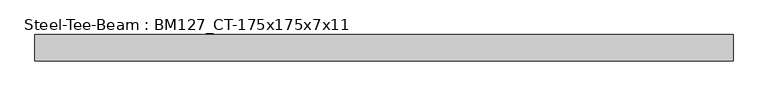
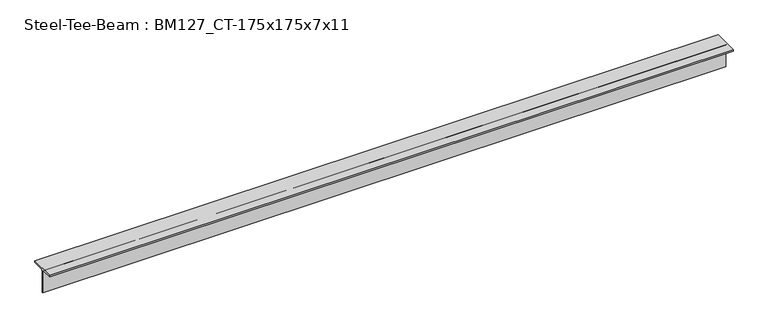
"""IFC4 building model written with IfcOpenShell, lengths in millimetres: beam geometry, Steel-Tee-Beam : BM127_CT-175x175x7x11."""

import ifcopenshell
import ifcopenshell.guid

model = None  # the IFC model being written
_history = None  # IfcOwnerHistory: only IFC2X3 demands one
_inside = {}  # id of a spatial element -> (the spatial element, [elements in it])
_under = {}  # id of a project, library or spatial element -> (it, [spatial elements below it])
_declared = {}  # id of a project -> (the project, [libraries it declares])
_typed = {}  # id of a type object -> (the type object, [elements of that type])
_made_of = {}  # id of a material, layer set ... -> (it, [elements and type objects made of it])


def new_model(schema):
    """Start an empty IFC model of exactly this schema.

    Asked for "IFC4X3", IfcOpenShell would pick the latest addendum, in which some entities
    have other attributes; the version numbers below select the first issue.
    IFC2X3 requires an IfcOwnerHistory on every rooted entity: one is made here for all.
    """
    global model, _history
    if schema == "IFC4X3":
        model = ifcopenshell.file(schema_version=(4, 3, 0, 0))
    else:
        model = ifcopenshell.file(schema=schema)
    _inside.clear()
    _under.clear()
    _declared.clear()
    _typed.clear()
    _made_of.clear()
    _history = None
    if model.schema == "IFC2X3":
        org = make("IfcOrganization", Name="unknown")
        user = make(
            "IfcPersonAndOrganization",
            ThePerson=make("IfcPerson", FamilyName="unknown"),
            TheOrganization=org,
        )
        app = make(
            "IfcApplication",
            ApplicationDeveloper=org,
            Version="unknown",
            ApplicationFullName="unknown",
            ApplicationIdentifier="unknown",
        )
        _history = make(
            "IfcOwnerHistory",
            OwningUser=user,
            OwningApplication=app,
            ChangeAction="ADDED",
            CreationDate=0,
        )
    return model


def make(cls, **values):
    """One entity of the class cls with the attributes given. An attribute that is None is left unset."""
    return model.create_entity(
        cls, **{name: value for name, value in values.items() if value is not None}
    )


def rooted(cls, **values):
    """An entity with a GlobalId (a new one), such as an element, a storey or a relation."""
    return make(cls, GlobalId=ifcopenshell.guid.new(), OwnerHistory=_history, **values)


def si_unit(unit_type, name, prefix=None):
    """IfcSIUnit, for example si_unit("LENGTHUNIT", "METRE", prefix="MILLI")."""
    return make("IfcSIUnit", UnitType=unit_type, Prefix=prefix, Name=name)


def assignment(units):
    """IfcUnitAssignment: the units of a project."""
    return None if units is None else make("IfcUnitAssignment", Units=units)


def point(xyz):
    """IfcCartesianPoint."""
    return None if xyz is None else make("IfcCartesianPoint", Coordinates=xyz)


def direction(xyz):
    """IfcDirection."""
    return None if xyz is None else make("IfcDirection", DirectionRatios=xyz)


def frame(location, z_axis=None, x_axis=None):
    """IfcAxis2Placement3D, a coordinate frame: its origin and axes. An axis left out is left unset."""
    return make(
        "IfcAxis2Placement3D",
        Location=point(location),
        Axis=direction(z_axis),
        RefDirection=direction(x_axis),
    )


def frame_2d(location, x_axis=None):
    """IfcAxis2Placement2D, a coordinate frame in the plane: its origin and x axis."""
    return make(
        "IfcAxis2Placement2D", Location=point(location), RefDirection=direction(x_axis)
    )


def origin():
    """The frame at (0, 0, 0) with its axes left unset."""
    return frame((0.0, 0.0, 0.0))


def place(relative_to, where):
    """IfcLocalPlacement: puts the frame where relative to a parent placement (None: the world)."""
    return make(
        "IfcLocalPlacement", PlacementRelTo=relative_to, RelativePlacement=where
    )


def context(
    kind, dimensions, precision=None, world=None, true_north=None, identifier=None
):
    """IfcGeometricRepresentationContext, for example the 3D "Model" context."""
    return make(
        "IfcGeometricRepresentationContext",
        ContextIdentifier=identifier,
        ContextType=kind,
        CoordinateSpaceDimension=dimensions,
        Precision=precision,
        WorldCoordinateSystem=world,
        TrueNorth=true_north,
    )


def project(units=None, contexts=None):
    """IfcProject with its units and contexts."""
    return rooted(
        "IfcProject",
        Name="project",
        RepresentationContexts=contexts,
        UnitsInContext=assignment(units),
    )


def spatial(cls, under=None, at=None, **own):
    """A site, building, storey or space (cls), placed at a placement, below another one or the project."""
    s = rooted(cls, ObjectPlacement=at, **own)
    if under is not None:
        _under.setdefault(under.id(), (under, []))[1].append(s)
    return s


def polyline(points):
    """IfcPolyline through the points."""
    return make("IfcPolyline", Points=[point(p) for p in points])


def circle_curve(where, radius):
    """IfcCircle in the frame where."""
    return make("IfcCircle", Position=where, Radius=radius)


def trimmed(basis, trim1, trim2, sense, master):
    """IfcTrimmedCurve: the piece of a basis curve between two trims."""
    return make(
        "IfcTrimmedCurve",
        BasisCurve=basis,
        Trim1=trim1,
        Trim2=trim2,
        SenseAgreement=sense,
        MasterRepresentation=master,
    )


def segment(curve, same_sense, transition):
    """IfcCompositeCurveSegment."""
    return make(
        "IfcCompositeCurveSegment",
        Transition=transition,
        SameSense=same_sense,
        ParentCurve=curve,
    )


def composite_curve(segments, self_intersect=None):
    """IfcCompositeCurve: segments joined end to end."""
    return make("IfcCompositeCurve", Segments=segments, SelfIntersect=self_intersect)


def outline(outer, holes=None, kind="AREA"):
    """IfcArbitraryClosedProfileDef: a profile drawn as a closed curve; with holes, ...WithVoids."""
    if holes is None:
        return make("IfcArbitraryClosedProfileDef", ProfileType=kind, OuterCurve=outer)
    return make(
        "IfcArbitraryProfileDefWithVoids",
        ProfileType=kind,
        OuterCurve=outer,
        InnerCurves=holes,
    )


def extrude(swept, where, along, depth):
    """IfcExtrudedAreaSolid: the profile swept, set in the frame where, extruded along a direction by depth."""
    return make(
        "IfcExtrudedAreaSolid",
        SweptArea=swept,
        Position=where,
        ExtrudedDirection=direction(along),
        Depth=depth,
    )


def shape(context_of_items, identifier, shape_type, items):
    """IfcShapeRepresentation: the items that make up one representation, for example the "Body"."""
    return make(
        "IfcShapeRepresentation",
        ContextOfItems=context_of_items,
        RepresentationIdentifier=identifier,
        RepresentationType=shape_type,
        Items=items,
    )


def source(mapping_origin, context_of_items, identifier, shape_type, items):
    """IfcRepresentationMap: a shape defined once, which mapped items show again and again."""
    return make(
        "IfcRepresentationMap",
        MappingOrigin=mapping_origin,
        MappedRepresentation=shape(context_of_items, identifier, shape_type, items),
    )


def transform(
    local_origin,
    x_axis=None,
    y_axis=None,
    z_axis=None,
    scale=None,
    scale2=None,
    scale3=None,
    uniform=True,
):
    """IfcCartesianTransformationOperator3D, or its non-uniform kind. x_axis, y_axis, z_axis: its Axis1, 2, 3."""
    if uniform:
        return make(
            "IfcCartesianTransformationOperator3D",
            Axis1=direction(x_axis),
            Axis2=direction(y_axis),
            LocalOrigin=point(local_origin),
            Scale=scale,
            Axis3=direction(z_axis),
        )
    return make(
        "IfcCartesianTransformationOperator3DnonUniform",
        Axis1=direction(x_axis),
        Axis2=direction(y_axis),
        LocalOrigin=point(local_origin),
        Scale=scale,
        Axis3=direction(z_axis),
        Scale2=scale2,
        Scale3=scale3,
    )


def mapped(mapping_source, mapping_target):
    """IfcMappedItem: shows the shape of a source again, moved by a transform."""
    return make(
        "IfcMappedItem", MappingSource=mapping_source, MappingTarget=mapping_target
    )


def made_of(thing, what):
    """Note that an element or type object is made of a material, layer set ...; save() writes the relation."""
    if what is not None:
        _made_of.setdefault(what.id(), (what, []))[1].append(thing)
    return thing


def element(
    cls,
    number,
    at=None,
    inside=None,
    cuts=None,
    type_object=None,
    material=None,
    context=None,
    identifier="Body",
    shape_type=None,
    held_by="IfcProductDefinitionShape",
    body=None,
    shapes=None,
    **own,
):
    """One element of the class cls, such as IfcWall. Its Tag is "e" and its number.

    at: its placement. inside: the storey or other place that contains it. cuts: it is an
    opening in that element (IfcRelVoidsElement). A single representation is given by context,
    identifier, shape_type and body (its items); several are given by shapes. held_by: the class
    of the entity that holds the representations. save() writes the other relations.
    """
    e = rooted(cls, Tag="e%d" % number, ObjectPlacement=at, **own)
    if body is not None:
        shapes = [shape(context, identifier, shape_type, body)]
    if shapes is not None:
        e.Representation = make(held_by, Representations=shapes)
    if inside is not None:
        _inside.setdefault(inside.id(), (inside, []))[1].append(e)
    if cuts is not None:
        rooted(
            "IfcRelVoidsElement", RelatingBuildingElement=cuts, RelatedOpeningElement=e
        )
    if type_object is not None:
        _typed.setdefault(type_object.id(), (type_object, []))[1].append(e)
    return made_of(e, material)


def aggregate(whole, parts):
    """IfcRelAggregates: a whole, such as a stair, and the parts it consists of."""
    return rooted("IfcRelAggregates", RelatingObject=whole, RelatedObjects=parts)


def save(model, path):
    """Write the relations noted so far, then the file.

    IfcRelAggregates (storeys below a building ...), IfcRelContainedInSpatialStructure (elements
    in a storey), IfcRelDefinesByType, IfcRelAssociatesMaterial and IfcRelDeclares: one each for
    every whole, place, type object, material and project.
    """
    for whole, parts in _under.values():
        aggregate(whole, parts)
    for where, things in _inside.values():
        rooted(
            "IfcRelContainedInSpatialStructure",
            RelatedElements=things,
            RelatingStructure=where,
        )
    for kind, things in _typed.values():
        rooted("IfcRelDefinesByType", RelatedObjects=things, RelatingType=kind)
    for what, things in _made_of.values():
        rooted("IfcRelAssociatesMaterial", RelatedObjects=things, RelatingMaterial=what)
    for by, libraries in _declared.values():
        rooted("IfcRelDeclares", RelatingContext=by, RelatedDefinitions=libraries)
    model.write(path)


def steel_tee_beam_bm127_ct_175x175x7x11_9f293f4f(model_context):
    return source(origin(), model_context, "Body", "SweptSolid", [
        extrude(outline(composite_curve([segment(polyline([(-87.5, 87.5), (87.5, 87.5), (87.5, 76.5), (17.5, 76.5)]), True, "CONTINUOUS"), segment(trimmed(circle_curve(frame_2d((17.5, 62.5)), 14.0), [point((17.5, 76.5))], [point((3.5, 62.5))], True, "CARTESIAN"), True, "CONTINUOUS"), segment(polyline([(3.5, 62.5), (3.5, -87.5), (-3.5, -87.5), (-3.5, 62.5)]), True, "CONTINUOUS"), segment(trimmed(circle_curve(frame_2d((-17.5, 62.5)), 14.0), [point((-3.5, 62.5))], [point((-17.5, 76.5))], True, "CARTESIAN"), True, "CONTINUOUS"), segment(polyline([(-17.5, 76.5), (-87.5, 76.5), (-87.5, 87.5)]), True, "CONTINUOUS")], self_intersect=False)), frame((-2276.3489916, 0.0, 0.0), z_axis=(1.0, 0.0, 0.0), x_axis=(0.0, 1.0, 0.0)), (0.0, 0.0, 1.0), 4641.606963),
    ])


if __name__ == "__main__":
    model = new_model("IFC4")
    model_context = context("Model", 3, world=origin())
    ifc_project = project(units=[si_unit("LENGTHUNIT", "METRE", prefix="MILLI")], contexts=[model_context])
    site = spatial("IfcSite", under=ifc_project)
    building = spatial("IfcBuilding", under=site)
    placement = place(None, origin())
    steel_tee_beam_bm127_ct_175x175x7x11_shape = steel_tee_beam_bm127_ct_175x175x7x11_9f293f4f(model_context)
    element("IfcBeam", 1, ObjectType="Steel-Tee-Beam : BM127_CT-175x175x7x11", at=placement, inside=building, context=model_context, shape_type="MappedRepresentation", body=[
        mapped(steel_tee_beam_bm127_ct_175x175x7x11_shape, transform((0.0, 0.0, 0.0), x_axis=(1.0, 0.0, 0.0), y_axis=(0.0, 1.0, 0.0), z_axis=(0.0, 0.0, 1.0))),
    ])
    save(model, "model.ifc")

# Revit data of these elements
# Type "Steel-Tee-Beam : BM127_CT-175x175x7x11"
#   Surface Area = 0.00 m²/m
#   Section Area = 31.57 cm²
#   Mass per Unit Length = 24.80 kg/m
#   Length [instance default] = 1524 mm
#   bf = 175 mm
#   d = 175 mm
#   k = 25 mm
#   kr = 14 mm
#   tf = 11 mm
#   tw = 7 mm
#   hec_material4 [instance default] = none
#   hec_material3 [instance default] = none
#   hec_material2 [instance default] = none
#   hec_material1 [instance default] = none
#   Structural Material [instance default] = Steel, 45-345
#   Assembly Code = ""
# Element 1 (IfcBeam, "Steel-Tee-Beam : BM127_CT-175x175x7x11")
#   hec_material3 = F01AC000-00002_Building/Shelter Fire Proofing Work_Intumescent Coating Type_1 hr. rating (UL 1709))
#   hec_material2 = S01AA010-00002_Main Steel Structure Fabrication Work_Shelter/Building_Steel Painting/Coating_for Fireproofed Steel Surface, Surface Preparation & Primer Coat
#   hec_material1 = S03AA029-00001_Main Steel Structure Erection Work_Shelter/Building_Light Steel
#   Structural Material = S01AA003-00001_Main Steel Structure Fabrication Work_Shelter/Building_Light Steel - Standard
#   Materials on its faces: "S01AA003-00001_Main Steel Structure Fabrication Work_Shelter/Building_Light Steel - Standard"
# Materials
#   "Steel, 45-345": class "Metal", colour RGB 189 187 185, transparency 0, Description = "Steel 345 MPa", Cost = 0
#   "S01AA003-00001_Main Steel Structure Fabrication Work_Shelter/Building_Light Steel - Standard": class "Metal", colour RGB 120 120 120, transparency 0, Comments = "(30KG/M>Weight)", Description = "Structural steel 50ksi", W00) Work Master Code = "S01AA003-00001", W01) Work Master_Lv1 = "Main Steel Structure Fabrication Work", W02) Work Master_Lv2 = "Shelter/Building", W03) Work Master_Spec.1 = "Light Steel - Standard (30KG/M>Weight)", Cost = 0
#   "F01AC000-00002_Building/Shelter Fire Proofing Work_Intumescent Coating Type_1 hr. rating (UL 1709))": class "Metal", colour RGB 255 128 128, transparency 0, Description = "Paint finished steel", W00) Work Master Code = "F01AC000-00002", W01) Work Master_Lv1 = "Building/Shelter Fire Proofing Work", W02) Work Master_Lv2 = "Intumescent Coating Type", W03) Work Master_Spec.1 = "1 hr. rating (UL 1709)", Cost = 0
#   "S01AA010-00002_Main Steel Structure Fabrication Work_Shelter/Building_Steel Painting/Coating_for Fireproofed Steel Surface, Surface Preparation & Primer Coat": class "Metal", colour RGB 120 120 120, transparency 0, Description = "Paint finished steel", W00) Work Master Code = "SS01AA010-00002", W01) Work Master_Lv1 = "Main Steel Structure Fabrication Work", W02) Work Master_Lv2 = "Shelter/Building", W03) Work Master_Spec.1 = "Steel Painting/Coating", W04) Work Master_Spec.2 = "for Fireproofed Steel Surface, Surface Preparation & Primer Coat", Cost = 0
#   "S03AA029-00001_Main Steel Structure Erection Work_Shelter/Building_Light Steel": class "Metal", colour RGB 120 120 120, transparency 0, Comments = "(30KG/M>Weight)", Description = "Structural steel 50ksi", W00) Work Master Code = "S03AA029-00001", W01) Work Master_Lv1 = "Main Steel Structure Erection Work", W02) Work Master_Lv2 = "Shelter/Building", W03) Work Master_Spec.1 = "Light Steel (30KG/M>Weight)", Cost = 0
